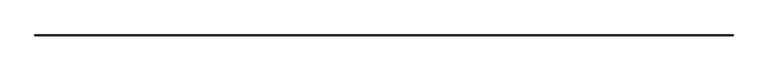
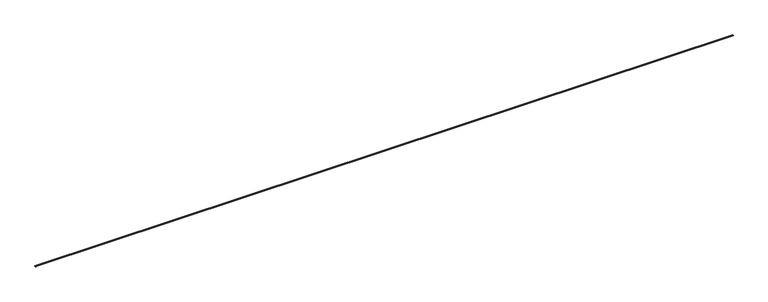
"""IFC4 building model written with IfcOpenShell, lengths in millimetres: proxy geometry, Generic Models 3:Generic Models 1:4:Generic Models 1:4 : Generic Models 3:Generic Models 1:300625:1:Generic Models 1:4:Generic Models 1:4 : Generic Models 3:Generic Models 1:300625:1 : Generic Models 3:Generic Models 1:4:Generic Models 1:4 : Generic Models 3:Generic Models 1:300625:338780:6 : Generic Models 3:Generic Models 1:4:Generic Models 1:4 : Generic Models 3:Generic Models 1:300625:1:Generic Models 1:4:Generic Models 1:4 : Generic Models 3:Generic Models 1:300625:1 : Generic Models 3:Generic Models 1:4:Generic Models 1:4 : Generic Models 3:Generic Models 1:300625:338780:317135."""

from ifc_helpers import new_model, si_unit, frame, origin, place, context, project, spatial, polyline, outline, extrude, source, transform, mapped, element, save


def generic_models_72f76a19(model_context):
    return source(origin(), model_context, "Body", "SweptSolid", [
        extrude(outline(polyline([(-568271.4513466, 8566.7287152), (-568277.6386894, 8566.7287152), (-568277.0920966, 8567.3801192), (-568276.8412704, 8568.3162152), (-568277.0920966, 8569.2523112), (-568277.6386894, 8569.9037152), (-568271.4513466, 8569.9037152), (-568271.9979394, 8569.2523112), (-568272.2487656, 8568.3162152), (-568271.9979394, 8567.3801192), (-568271.4513466, 8566.7287152)])), frame((591306.0367242, 0.0, 0.0), z_axis=(1.0, 0.0, 0.0), x_axis=(0.0, 1.0, 0.0)), (0.0, 0.0, 1.0), 4876.8),
    ])


if __name__ == "__main__":
    model = new_model("IFC4")
    model_context = context("Model", 3, world=origin())
    ifc_project = project(units=[si_unit("LENGTHUNIT", "METRE", prefix="MILLI")], contexts=[model_context])
    site = spatial("IfcSite", under=ifc_project)
    building = spatial("IfcBuilding", under=site)
    placement = place(None, origin())
    generic_models_shape = generic_models_72f76a19(model_context)
    element("IfcBuildingElementProxy", 1, Name="Generic Models 3:Generic Models 1:4:Generic Models 1:4 : Generic Models 3:Generic Models 1:300625:1:Generic Models 1:4:Generic Models 1:4 : Generic Models 3:Generic Models 1:300625:1 : Generic Models 3:Generic Models 1:4:Generic Models 1:4 : Generic Models 3:Generic Models 1:300625:338780:6 : Generic Models 3:Generic Models 1:4:Generic Models 1:4 : Generic Models 3:Generic Models 1:300625:1:Generic Models 1:4:Generic Models 1:4 : Generic Models 3:Generic Models 1:300625:1 : Generic Models 3:Generic Models 1:4:Generic Models 1:4 : Generic Models 3:Generic Models 1:300625:338780:317135", ObjectType="Generic Models 3:Generic Models 1:4:Generic Models 1:4 : Generic Models 3:Generic Models 1:300625:1:Generic Models 1:4:Generic Models 1:4 : Generic Models 3:Generic Models 1:300625:1 : Generic Models 3:Generic Models 1:4:Generic Models 1:4 : Generic Models 3:Generic Models 1:300625:338780:6 : Generic Models 3:Generic Models 1:4:Generic Models 1:4 : Generic Models 3:Generic Models 1:300625:1:Generic Models 1:4:Generic Models 1:4 : Generic Models 3:Generic Models 1:300625:1 : Generic Models 3:Generic Models 1:4:Generic Models 1:4 : Generic Models 3:Generic Models 1:300625:338780:317135", at=placement, inside=building, context=model_context, shape_type="MappedRepresentation", body=[
        mapped(generic_models_shape, transform((0.0, 0.0, 0.0), x_axis=(1.0, 0.0, 0.0), y_axis=(0.0, 1.0, 0.0), z_axis=(0.0, 0.0, 1.0))),
    ])
    save(model, "model.ifc")

# Revit data of these elements
# Type "Generic Models 3:Generic Models 1:4:Generic Models 1:4 : Generic Models 3:Generic Models 1:300625:1:Generic Models 1:4:Generic Models 1:4 : Generic Models 3:Generic Models 1:300625:1 : Generic Models 3:Generic Models 1:4:Generic Models 1:4 : Generic Models 3:Generic Models 1:300625:338780:6 : Generic Models 3:Generic Models 1:4:Generic Models 1:4 : Generic Models 3:Generic Models 1:300625:1:Generic Models 1:4:Generic Models 1:4 : Generic Models 3:Generic Models 1:300625:1 : Generic Models 3:Generic Models 1:4:Generic Models 1:4 : Generic Models 3:Generic Models 1:300625:338780:317135"
#   NameOverride = "Generic Models 3:Generic Models 1:4:Generic Models 1:4 : Generic Models 3:Generic Models 1:300625:1:Generic Models 1:4:Generic Models 1:4 : Generic Models 3:Generic Models 1:300625:1 : Generic Models 3:Generic Models 1:4:Generic Models 1:4 : Generic Models 3:Generic Models 1:300625:338780:317135"
#   ObjectTypeOverride = "Generic Models 1:4:Generic Models 1:4 : Generic Models 3:Generic Models 1:300625:1 : Generic Models 3:Generic Models 1:4:Generic Models 1:4 : Generic Models 3:Generic Models 1:300625:338780"
#   Reference = "Generic Models 1"
#   Tag = "317135"
# Element 1 (IfcBuildingElementProxy, "Generic Models 3:Generic Models 1:4:Generic Models 1:4 : Generic Models 3:Generic Models 1:300625:1:Generic Models 1:4:Generic Models 1:4 : Generic Models 3:Generic Models 1:300625:1 : Generic Models 3:Generic Models 1:4:Generic Models 1:4 : Generic Models 3:Generic Models 1:300625:338780:6 : Generic Models 3:Generic Models 1:4:Generic Models 1:4 : Generic Models 3:Generic Models 1:300625:1:Generic Models 1:4:Generic Models 1:4 : Generic Models 3:Generic Models 1:300625:1 : Generic Models 3:Generic Models 1:4:Generic Models 1:4 : Generic Models 3:Generic Models 1:300625:338780:317135")
#   Materials on its faces: "SEALANT & BACKER ROD, IF NECESSARY"
# Materials
#   "SEALANT & BACKER ROD, IF NECESSARY": class "Unassigned", colour RGB 120 120 120, transparency 0, Cost = 0
